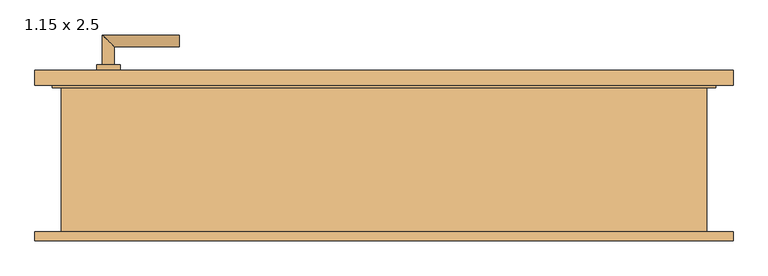
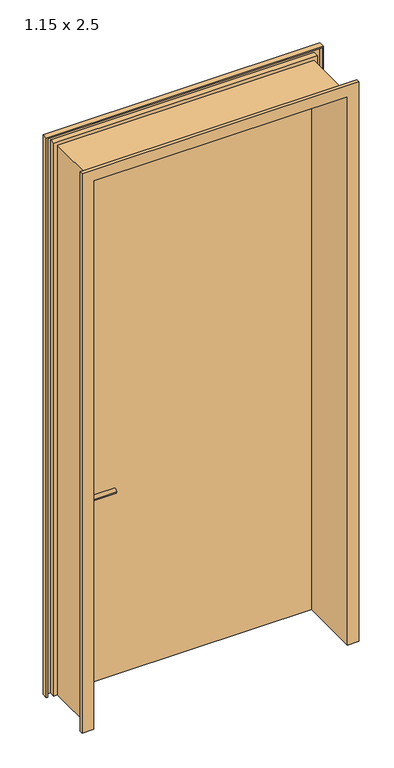
"""IFC4 building model written with IfcOpenShell, lengths in millimetres: door geometry, Drehflügel 1-flg - Stahlzarge : 1.15 x 2.5."""

from ifc_helpers import new_model, si_unit, point, frame, frame_2d, origin, place, context, project, spatial, polyline, circle_curve, ellipse_curve, trimmed, segment, composite_curve, outline, extrude, faceted_brep, source, transform, mapped, element, save
from ifc_brep_helpers import plane_surface, cylinder_surface, advanced_brep


def door_1_15_x_2_5_fbf7b17d(model_context):
    return source(origin(), model_context, "Body", "SolidModel", [
        advanced_brep(
        [(-477.5, 113.9346141, 901.0), (-457.5, 113.9346141, 901.0), (-477.5, 43.9346141, 901.0), (-457.5, 63.9346141, 901.0), (-347.5, 43.9346141, 901.0), (-347.5, 63.9346141, 901.0)],
        [
            (0, 1, circle_curve(frame((-467.5, 113.9346141, 901.0), z_axis=(0.0, 1.0, 0.0), x_axis=(1.0, 0.0, 0.0)), 10.0)),
            (1, 0, circle_curve(frame((-467.5, 113.9346141, 901.0), z_axis=(0.0, 1.0, 0.0), x_axis=(1.0, 0.0, 0.0)), 10.0)),
            (0, 2),
            (2, 3, ellipse_curve(frame((-467.5, 53.9346141, 901.0), z_axis=(-0.7071067811865385, 0.7071067811865565, 0.0), x_axis=(0.7071067811865563, 0.7071067811865386, 0.0)), 14.1421356, 10.0)),
            (3, 1),
            (3, 2, ellipse_curve(frame((-467.5, 53.9346141, 901.0), z_axis=(-0.7071067811865385, 0.7071067811865565, 0.0), x_axis=(0.7071067811865563, 0.7071067811865386, 0.0)), 14.1421356, 10.0)),
            (4, 5, circle_curve(frame((-347.5, 53.9346141, 901.0), z_axis=(1.0, 0.0, 0.0), x_axis=(0.0, 1.0, 0.0)), 10.0)),
            (5, 4, circle_curve(frame((-347.5, 53.9346141, 901.0), z_axis=(1.0, 0.0, 0.0), x_axis=(0.0, 1.0, 0.0)), 10.0)),
            (2, 4),
            (5, 3),
        ],
        [
            plane_surface(frame((-467.5, 113.9346141, -386.7526403), z_axis=(0.0, 1.0, 0.0), x_axis=(0.0, 0.0, 1.0))),
            cylinder_surface(frame((-467.5, 113.9346141, 901.0), z_axis=(0.0, 1.0, 0.0), x_axis=(1.0, 0.0, 0.0)), 10.0),
            plane_surface(frame((-347.5, 53.9346141, -386.7526403), z_axis=(1.0, 0.0, 0.0), x_axis=(0.0, 0.0, 1.0))),
            cylinder_surface(frame((-467.5, 53.9346141, 901.0), z_axis=(-1.0, 0.0, 0.0), x_axis=(0.0, 1.0, 0.0)), 10.0),
        ],
        [
            (0, [[1, 2]]),
            (1, [[-1, 3, 4, 5]]),
            (1, [[-2, -5, 6, -3]]),
            (2, [[7, 8]]),
            (3, [[-4, 9, -8, 10]]),
            (3, [[-6, -10, -7, -9]]),
        ],
    ),
        advanced_brep(
        [(-457.5, 173.9346141, 901.0), (-477.5, 173.9346141, 901.0), (-457.5, 203.9346141, 901.0), (-477.5, 223.9346141, 901.0), (-347.5, 203.9346141, 901.0), (-347.5, 223.9346141, 901.0)],
        [
            (0, 1, circle_curve(frame((-467.5, 173.9346141, 901.0), z_axis=(0.0, -1.0, 0.0), x_axis=(-1.0, 0.0, 0.0)), 10.0)),
            (1, 0, circle_curve(frame((-467.5, 173.9346141, 901.0), z_axis=(0.0, -1.0, 0.0), x_axis=(-1.0, 0.0, 0.0)), 10.0)),
            (0, 2),
            (2, 3, ellipse_curve(frame((-467.5, 213.9346141, 901.0), z_axis=(-0.7071067811865475, -0.7071067811865475, 0.0), x_axis=(0.7071067811865474, -0.7071067811865476, 0.0)), 14.1421356, 10.0)),
            (3, 1),
            (3, 2, ellipse_curve(frame((-467.5, 213.9346141, 901.0), z_axis=(-0.7071067811865475, -0.7071067811865475, 0.0), x_axis=(0.7071067811865474, -0.7071067811865476, 0.0)), 14.1421356, 10.0)),
            (4, 5, circle_curve(frame((-347.5, 213.9346141, 901.0), z_axis=(1.0, 0.0, 0.0), x_axis=(0.0, 1.0, 0.0)), 10.0)),
            (5, 4, circle_curve(frame((-347.5, 213.9346141, 901.0), z_axis=(1.0, 0.0, 0.0), x_axis=(0.0, 1.0, 0.0)), 10.0)),
            (2, 4),
            (5, 3),
        ],
        [
            plane_surface(frame((-467.5, 173.9346141, -386.7526403), z_axis=(0.0, -1.0, 0.0), x_axis=(0.0, 0.0, 1.0))),
            cylinder_surface(frame((-467.5, 173.9346141, 901.0), z_axis=(0.0, -1.0, 0.0), x_axis=(-1.0, 0.0, 0.0)), 10.0),
            plane_surface(frame((-347.5, 213.9346141, -386.7526403), z_axis=(1.0, 0.0, 0.0), x_axis=(0.0, 0.0, 1.0))),
            cylinder_surface(frame((-467.5, 213.9346141, 901.0), z_axis=(-1.0, 0.0, 0.0), x_axis=(0.0, 1.0, 0.0)), 10.0),
        ],
        [
            (0, [[1, 2]]),
            (1, [[-1, 3, 4, 5]]),
            (1, [[-2, -5, 6, -3]]),
            (2, [[7, 8]]),
            (3, [[-4, 9, -8, 10]]),
            (3, [[-6, -10, -7, -9]]),
        ],
    ),
        extrude(outline(composite_curve([segment(trimmed(circle_curve(frame_2d((901.0, -467.5)), 20.0), [point((901.0, -487.5))], [point((901.0, -447.5))], False, "CARTESIAN"), True, "CONTINUOUS"), segment(trimmed(circle_curve(frame_2d((901.0, -467.5)), 20.0), [point((901.0, -447.5))], [point((901.0, -487.5))], False, "CARTESIAN"), True, "CONTINUOUS")], self_intersect=False)), frame((0.0, 103.9346141, 0.0), z_axis=(0.0, 1.0, 0.0), x_axis=(0.0, 0.0, 1.0)), (0.0, 0.0, 1.0), 10.0),
        extrude(outline(composite_curve([segment(trimmed(circle_curve(frame_2d((901.0, -467.5)), 20.0), [point((901.0, -487.5))], [point((901.0, -447.5))], False, "CARTESIAN"), True, "CONTINUOUS"), segment(trimmed(circle_curve(frame_2d((901.0, -467.5)), 20.0), [point((901.0, -447.5))], [point((901.0, -487.5))], False, "CARTESIAN"), True, "CONTINUOUS")], self_intersect=False)), frame((0.0, 163.9346141, 0.0), z_axis=(0.0, 1.0, 0.0), x_axis=(0.0, 0.0, 1.0)), (0.0, 0.0, 1.0), 10.0),
        extrude(outline(polyline([(557.5, 138.9346141), (-557.5, 138.9346141), (-557.5, 163.9346141), (557.5, 163.9346141), (557.5, 138.9346141)])), frame((0.0, 0.0, 1.0), z_axis=(0.0, 0.0, 1.0), x_axis=(1.0, 0.0, 0.0)), (0.0, 0.0, 1.0), 2490.0),
        faceted_brep([(591.9603207, -125.0653859, 1.0), (542.5, -125.0653859, 1.0), (542.5, 138.9346141, 1.0), (557.5, 138.9346141, 1.0), (557.5, 163.9346141, 1.0), (591.9603207, 163.9346141, 1.0), (591.9603207, 138.9346141, 1.0), (586.9603207, 138.9346141, 1.0), (586.9603207, 158.9346141, 1.0), (562.5, 158.9346141, 1.0), (562.5, 133.9346141, 1.0), (547.5, 133.9346141, 1.0), (547.5, -120.0653859, 1.0), (586.9603207, -120.0653859, 1.0), (586.9603207, -110.0653859, 1.0), (591.9603207, -110.0653859, 1.0), (591.9603207, -125.0653859, 2525.4603207), (-591.9603207, -125.0653859, 2525.4603207), (-591.9603207, -125.0653859, 1.0), (-542.5, -125.0653859, 1.0), (-542.5, -125.0653859, 2476.0), (542.5, -125.0653859, 2476.0), (542.5, 138.9346141, 2476.0), (-542.5, 138.9346141, 2476.0), (-542.5, 138.9346141, 1.0), (-557.5, 138.9346141, 1.0), (-557.5, 138.9346141, 2491.0), (557.5, 138.9346141, 2491.0), (557.5, 163.9346141, 2491.0), (-557.5, 163.9346141, 2491.0), (-557.5, 163.9346141, 1.0), (-591.9603207, 163.9346141, 1.0), (-591.9603207, 163.9346141, 2525.4603207), (591.9603207, 163.9346141, 2525.4603207), (591.9603207, 138.9346141, 2525.4603207), (-591.9603207, 138.9346141, 2525.4603207), (-591.9603207, 138.9346141, 1.0), (-586.9603207, 138.9346141, 1.0), (-586.9603207, 138.9346141, 2520.4603207), (586.9603207, 138.9346141, 2520.4603207), (586.9603207, 158.9346141, 2520.4603207), (-586.9603207, 158.9346141, 2520.4603207), (-586.9603207, 158.9346141, 1.0), (-562.5, 158.9346141, 1.0), (-562.5, 158.9346141, 2496.0), (562.5, 158.9346141, 2496.0), (562.5, 133.9346141, 2496.0), (-562.5, 133.9346141, 2496.0), (-562.5, 133.9346141, 1.0), (-547.5, 133.9346141, 1.0), (-547.5, 133.9346141, 2481.0), (547.5, 133.9346141, 2481.0), (547.5, -120.0653859, 2481.0), (-547.5, -120.0653859, 2481.0), (-547.5, -120.0653859, 1.0), (-586.9603207, -120.0653859, 1.0), (-586.9603207, -120.0653859, 2520.4603207), (586.9603207, -120.0653859, 2520.4603207), (586.9603207, -110.0653859, 2520.4603207), (-586.9603207, -110.0653859, 2520.4603207), (-586.9603207, -110.0653859, 1.0), (-591.9603207, -110.0653859, 1.0), (-591.9603207, -110.0653859, 2525.4603207), (591.9603207, -110.0653859, 2525.4603207)], [[[0, 1, 2, 3, 4, 5, 6, 7, 8, 9, 10, 11, 12, 13, 14, 15]], [[1, 0, 16, 17, 18, 19, 20, 21]], [[2, 1, 21, 22]], [[3, 2, 22, 23, 24, 25, 26, 27]], [[4, 3, 27, 28]], [[5, 4, 28, 29, 30, 31, 32, 33]], [[6, 5, 33, 34]], [[7, 6, 34, 35, 36, 37, 38, 39]], [[8, 7, 39, 40]], [[9, 8, 40, 41, 42, 43, 44, 45]], [[10, 9, 45, 46]], [[11, 10, 46, 47, 48, 49, 50, 51]], [[12, 11, 51, 52]], [[13, 12, 52, 53, 54, 55, 56, 57]], [[14, 13, 57, 58]], [[15, 14, 58, 59, 60, 61, 62, 63]], [[0, 15, 63, 16]], [[17, 62, 61, 18]], [[18, 61, 60, 55, 54, 49, 48, 43, 42, 37, 36, 31, 30, 25, 24, 19]], [[23, 20, 19, 24]], [[29, 26, 25, 30]], [[35, 32, 31, 36]], [[41, 38, 37, 42]], [[47, 44, 43, 48]], [[53, 50, 49, 54]], [[59, 56, 55, 60]], [[22, 21, 20, 23]], [[28, 27, 26, 29]], [[34, 33, 32, 35]], [[40, 39, 38, 41]], [[46, 45, 44, 47]], [[52, 51, 50, 53]], [[58, 57, 56, 59]], [[16, 63, 62, 17]]]),
    ])


if __name__ == "__main__":
    model = new_model("IFC4")
    model_context = context("Model", 3, world=origin())
    ifc_project = project(units=[si_unit("LENGTHUNIT", "METRE", prefix="MILLI")], contexts=[model_context])
    site = spatial("IfcSite", under=ifc_project)
    building = spatial("IfcBuilding", under=site)
    placement = place(None, origin())
    door_1_15_x_2_5_shape = door_1_15_x_2_5_fbf7b17d(model_context)
    element("IfcDoor", 1, ObjectType="Drehflügel 1-flg - Stahlzarge : 1.15 x 2.5", at=placement, inside=building, context=model_context, shape_type="MappedRepresentation", body=[
        mapped(door_1_15_x_2_5_shape, transform((0.0, 0.0, 0.0), x_axis=(1.0, 0.0, 0.0), y_axis=(0.0, 1.0, 0.0), z_axis=(0.0, 0.0, 1.0))),
    ])
    save(model, "model.ifc")

# Revit data of these elements
# Type "Drehflügel 1-flg - Stahlzarge : 1.15 x 2.5"
#   Type Mark = "21"
#   Operation = "SingleSwingRight"
#   Keynote = "16.03"
#   Analytic Construction = "Metall"
#   Thermal Resistance (R) = 0.270117 (m²·K)/W
#   Heat Transfer Coefficient (U) = 3.7021 W/(m²·K)
#   Rough Width = 1.135 m
#   Rough Height [instance default] = 2.600 m
#   Höhe Türgriff [instance default] = 0.900 m
#   Height = 2.500 m
#   Fußbodenaufbau [instance default] = 0.100 m
#   Width = 1.135 m
#   Sichtbarkeit Sturzlinien [instance default] = yes
#   Türgriff auswählen [instance default] = element 221079
#   Türgriff [instance default] = none
#   Türflügel [instance default] = none
#   Rahmen/Pfosten [instance default] = Metall - Lackiert - Grau
#   Visual Light Transmittance = 0
#   Solar Heat Gain Coefficient = 0
#   Function = (empty or 0)
#   Wall Closure = (empty or 0)
# Element 1 (IfcDoor, "Drehflügel 1-flg - Stahlzarge : 1.15 x 2.5")
#   Rough Height = 2.501 m
#   Fußbodenaufbau = 0.001 m
#   Materials on its faces: "Metall - Lackiert - Grau", "Metall - Chrom", "Holz - Birke"
# Materials
#   "Metall - Lackiert - Grau": class "Farbe 1", colour RGB 98 98 98, transparency 0, Cost = 0
#   "Metall - Chrom": class "Metall", colour RGB 247 247 247, transparency 0, Cost = 0
#   "Holz - Birke": class "Holz", colour RGB 213 164 103, transparency 0, Cost = 0
